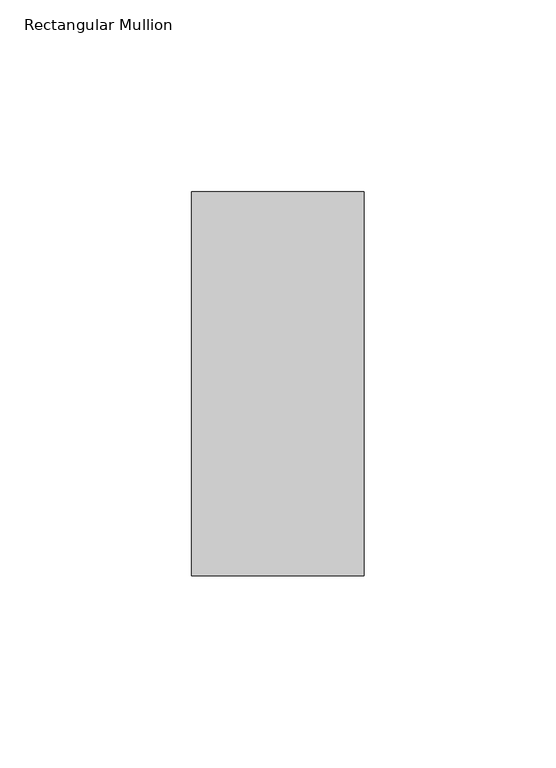
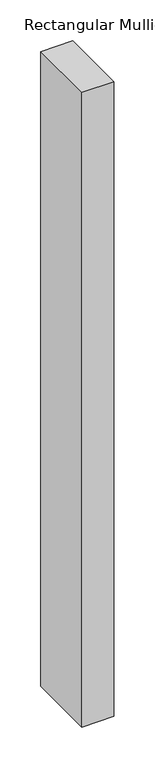
"""IFC4 building model written with IfcOpenShell, lengths in millimetres: member geometry, Rectangular Mullion : 알루미늄_Rectangular Cap_100 x 45."""

from ifc_helpers import new_model, si_unit, frame, origin, place, context, project, spatial, polyline, outline, extrude, source, transform, mapped, element, save


def rectangular_mullion_0724173d(model_context):
    return source(origin(), model_context, "Body", "SweptSolid", [
        extrude(outline(polyline([(0.0, 50.0), (0.0, -50.0), (-45.0, -50.0), (-45.0, 50.0), (0.0, 50.0)])), frame((0.0, 0.0, -945.0), z_axis=(0.0, 0.0, 1.0), x_axis=(1.0, 0.0, 0.0)), (0.0, 0.0, 1.0), 945.0),
    ])


if __name__ == "__main__":
    model = new_model("IFC4")
    model_context = context("Model", 3, world=origin())
    ifc_project = project(units=[si_unit("LENGTHUNIT", "METRE", prefix="MILLI")], contexts=[model_context])
    site = spatial("IfcSite", under=ifc_project)
    building = spatial("IfcBuilding", under=site)
    placement = place(None, origin())
    rectangular_mullion_shape = rectangular_mullion_0724173d(model_context)
    element("IfcMember", 1, ObjectType="Rectangular Mullion : 알루미늄_Rectangular Cap_100 x 45", at=placement, inside=building, context=model_context, shape_type="MappedRepresentation", body=[
        mapped(rectangular_mullion_shape, transform((0.0, 0.0, 0.0), x_axis=(1.0, 0.0, 0.0), y_axis=(0.0, 1.0, 0.0), z_axis=(0.0, 0.0, 1.0))),
    ])
    save(model, "model.ifc")

# Revit data of these elements
# Type "Rectangular Mullion : 알루미늄_Rectangular Cap_100 x 45"
#   built-in parameter 1007304 = 0.328084 (stored number, unit not read)
#   built-in parameter 1007301 = 0.0738189 (stored number, unit not read)
#   built-in parameter 1007300 = 0.0738189 (stored number, unit not read)
# Element 1 (IfcMember, "Rectangular Mullion : 알루미늄_Rectangular Cap_100 x 45")
#   Materials on its faces: "00_Metal_Stainless Steel"
# Materials
#   "00_Metal_Stainless Steel": class "Metal", colour RGB 148 148 148, transparency 0, Description = "Steel", Cost = 0
